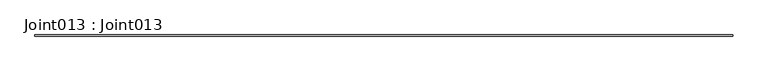
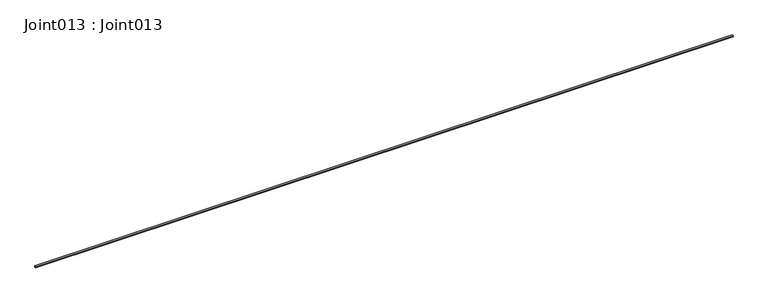
"""IFC4 building model written with IfcOpenShell, lengths in millimetres: proxy geometry, Joint013 : Joint013."""

from ifc_helpers import new_model, si_unit, point, frame, frame_2d, origin, place, context, project, spatial, polyline, circle_curve, trimmed, segment, composite_curve, outline, extrude, source, transform, mapped, element, save


def joint013_joint013_c31ac743(model_context):
    return source(origin(), model_context, "Body", "SweptSolid", [
        extrude(outline(composite_curve([segment(trimmed(circle_curve(frame_2d((-4379.145124, 41079.1499062)), 5.4132205), [point((-4377.546792, 41073.9780312))], [point((-4380.743456, 41073.9780312))], False, "CARTESIAN"), True, "CONTINUOUS"), segment(polyline([(-4380.743456, 41073.9780312), (-4380.743456, 41077.896)]), True, "CONTINUOUS"), segment(trimmed(circle_curve(frame_2d((-4379.145124, 41083.067875)), 5.4132205), [point((-4380.743456, 41077.896))], [point((-4377.546792, 41077.896))], True, "CARTESIAN"), True, "CONTINUOUS"), segment(polyline([(-4377.546792, 41077.896), (-4377.546792, 41073.9780312)]), True, "CONTINUOUS")], self_intersect=False)), frame((12383.0178845, 0.0, 0.0), z_axis=(1.0, 0.0, 0.0), x_axis=(0.0, 1.0, 0.0)), (0.0, 0.0, 1.0), 2000.0),
    ])


if __name__ == "__main__":
    model = new_model("IFC4")
    model_context = context("Model", 3, world=origin())
    ifc_project = project(units=[si_unit("LENGTHUNIT", "METRE", prefix="MILLI")], contexts=[model_context])
    site = spatial("IfcSite", under=ifc_project)
    building = spatial("IfcBuilding", under=site)
    placement = place(None, origin())
    joint013_joint013_shape = joint013_joint013_c31ac743(model_context)
    element("IfcBuildingElementProxy", 1, Name="Joint013 : Joint013", ObjectType="Joint013 : Joint013", at=placement, inside=building, context=model_context, shape_type="MappedRepresentation", body=[
        mapped(joint013_joint013_shape, transform((0.0, 0.0, 0.0), x_axis=(1.0, 0.0, 0.0), y_axis=(0.0, 1.0, 0.0), z_axis=(0.0, 0.0, 1.0))),
    ])
    save(model, "model.ifc")

# Revit data of these elements
# Type "Joint013 : Joint013"
#   NameOverride = "Joint013"
# Element 1 (IfcBuildingElementProxy, "Joint013 : Joint013")
#   Materials on its faces: "SILICON JOINT"
# Materials
#   "SILICON JOINT": class "Unassigned", colour RGB 150 184 127, transparency 0
